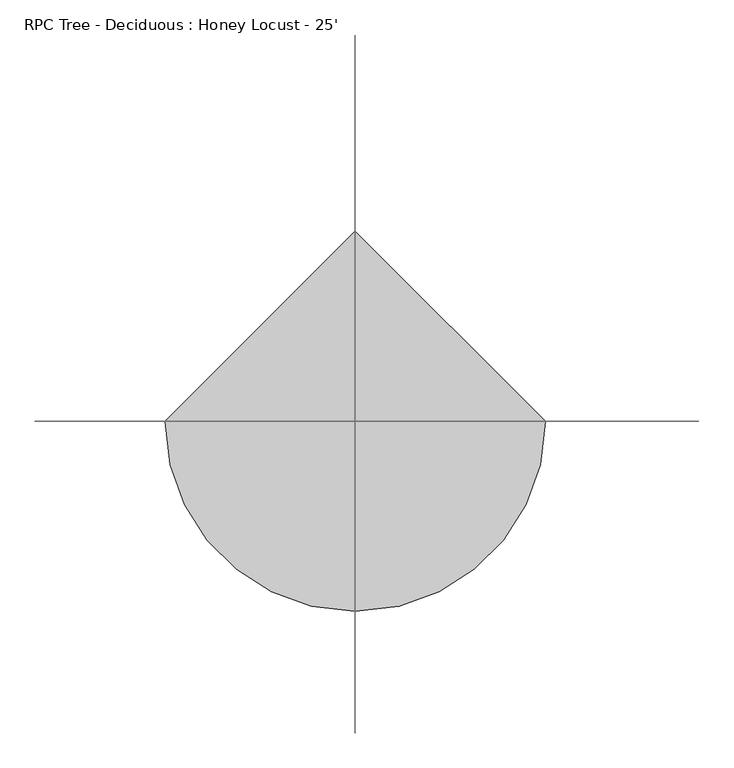
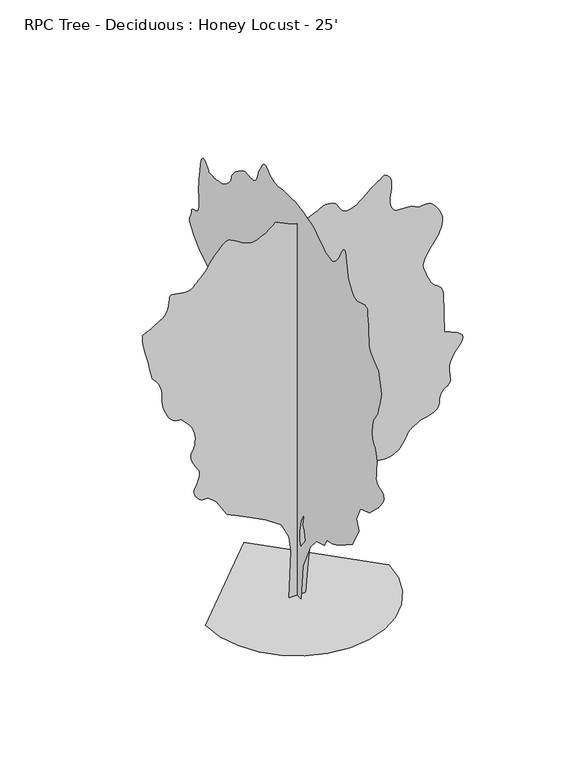
"""IFC4 building model written with IfcOpenShell, lengths in millimetres: geographic element geometry, RPC Tree - Deciduous : Honey Locust - 25'."""

from ifc_helpers import new_model, si_unit, origin, place, context, project, spatial, triangles, source, transform, mapped, element, save


def rpc_tree_deciduous_honey_locust_25_cc46a1f1(model_context):
    return source(origin(), model_context, "Body", "Tessellation", [
        triangles([(0.0017564, 138.2462219, 0.0), (0.0017564, -127.0105432, 0.0), (0.0017564, -184.6753374, 668.9082985), (0.0017564, -426.8668951, 1176.3566122), (0.0017564, -611.3926231, 1395.4822632), (0.0017564, -865.1155083, 1476.2135273), (0.0017564, -934.3152088, 1614.6078415), (0.0017564, -1118.8409369, 1660.7391827), (0.0017564, -1168.1321142, 1679.0297813), (0.0017564, -1234.9772346, 1712.4509972), (0.0017564, -1316.4476978, 1758.4833618), (0.0017564, -1409.6173016, 1814.6021748), (0.0017564, -1511.5651485, 1878.2849155), (0.0017564, -1619.3626385, 1947.0122612), (0.0017564, -1730.0862579, 2018.2590752), (0.0017564, -1937.6776566, 2398.8447109), (0.0017564, -1856.9463924, 2583.3806854), (0.0017564, -1983.8091431, 2848.632518), (0.0017564, -2272.1318058, 2952.4168808), (0.0017564, -2537.389016, 3206.1371498), (0.0017564, -2543.9089668, 3214.0110878), (0.0017564, -2561.3334846, 3235.1946785), (0.0017564, -2586.4031754, 3266.0558762), (0.0017564, -2615.9435234, 3302.9873428), (0.0017564, -2646.6774033, 3342.3317436), (0.0017564, -2675.3794304, 3380.4573235), (0.0017564, -2698.8489281, 3413.7311646), (0.0017564, -2714.4444878, 3444.5414932), (0.0017564, -2721.9882133, 3476.5453537), (0.0017564, -2721.8358971, 3508.1684235), (0.0017564, -2714.4444878, 3537.73377), (0.0017564, -2700.1950668, 3563.6926506), (0.0017564, -2679.4940048, 3584.4190018), (0.0017564, -2652.7226738, 3598.2620522), (0.0017564, -2621.3536583, 3608.345739), (0.0017564, -2588.1556847, 3619.6488281), (0.0017564, -2555.5675575, 3633.3648514), (0.0017564, -2526.024884, 3650.7129204), (0.0017564, -2501.9153091, 3672.9124374), (0.0017564, -2485.67444, 3701.157225), (0.0017564, -2479.7233498, 3736.6663948), (0.0017564, -2481.5749809, 3780.2273987), (0.0017564, -2486.0453476, 3831.0780739), (0.0017564, -2491.5266991, 3887.9740196), (0.0017564, -2496.4008202, 3949.6961243), (0.0017564, -2499.0579254, 4015.0755638), (0.0017564, -2497.8818344, 4082.8426483), (0.0017564, -2491.2575294, 4151.8544243), (0.0017564, -2477.5720276, 4213.7541344), (0.0017564, -2458.0368828, 4262.9284584), (0.0017564, -2435.2733013, 4302.24757), (0.0017564, -2411.9053963, 4334.4801956), (0.0017564, -2390.5542286, 4362.4965088), (0.0017564, -2373.8434753, 4389.0902344), (0.0017564, -2364.3947788, 4417.1062569), (0.0017564, -2359.5864967, 4450.1263344), (0.0017564, -2355.5860142, 4489.1913918), (0.0017564, -2353.1983692, 4533.3113731), (0.0017564, -2353.2315067, 4581.4694801), (0.0017564, -2356.4927902, 4632.6250786), (0.0017564, -2363.7901646, 4685.8128204), (0.0017564, -2375.9288132, 4740.016198), (0.0017564, -2392.0679443, 4787.9461212), (0.0017564, -2410.4271435, 4825.3601166), (0.0017564, -2430.3991802, 4855.916391), (0.0017564, -2451.3794403, 4883.2722794), (0.0017564, -2472.7636002, 4911.0089584), (0.0017564, -2493.9471909, 4942.7843445), (0.0017564, -2514.3232727, 4982.2051941), (0.0017564, -2534.0944496, 5031.4045166), (0.0017564, -2553.8659172, 5089.0626251), (0.0017564, -2573.6269203, 5153.8075104), (0.0017564, -2593.4135033, 5224.1654251), (0.0017564, -2613.1747971, 5298.7905212), (0.0017564, -2632.9360909, 5376.2096329), (0.0017564, -2652.7226738, 5455.0763306), (0.0017564, -2548.9127312, 5835.6443802), (0.0017564, -2410.52612, 5939.4537415), (0.0017564, -2376.165136, 5966.8602081), (0.0017564, -2343.2136589, 5995.5625259), (0.0017564, -2313.0867188, 6026.9059616), (0.0017564, -2287.1965839, 6062.1863663), (0.0017564, -2266.9553776, 6102.6995911), (0.0017564, -2253.772752, 6149.7659042), (0.0017564, -2249.0662079, 6204.705574), (0.0017564, -2247.7225399, 6269.3992996), (0.0017564, -2243.9556187, 6343.7709229), (0.0017564, -2238.1721054, 6426.2187973), (0.0017564, -2230.7756092, 6515.1186035), (0.0017564, -2222.1675591, 6608.8704391), (0.0017564, -2212.7518547, 6705.8220795), (0.0017564, -2202.9347214, 6804.4247818), (0.0017564, -2185.5179066, 6814.1270966), (0.0017564, -2167.3950302, 6822.8393555), (0.0017564, -2147.8598854, 6829.5453415), (0.0017564, -2126.2064106, 6833.2026764), (0.0017564, -2101.7285442, 6832.8218857), (0.0017564, -2073.7199341, 6827.4117508), (0.0017564, -2041.4746639, 6815.9560547), (0.0017564, -2006.8748863, 6801.3255524), (0.0017564, -1972.2775795, 6787.914743), (0.0017564, -1937.6776566, 6776.9165771), (0.0017564, -1903.077879, 6769.5501663), (0.0017564, -1868.4805721, 6767.0357849), (0.0017564, -1833.8806492, 6770.5663834), (0.0017564, -1799.2833424, 6781.3616547), (0.0017564, -1765.6919334, 6801.5546082), (0.0017564, -1733.9191635, 6831.4504578), (0.0017564, -1703.6576385, 6869.42314), (0.0017564, -1674.6050514, 6913.8221741), (0.0017564, -1646.4618565, 6963.0982361), (0.0017564, -1618.9257465, 7015.5746841), (0.0017564, -1591.689473, 7069.6766144), (0.0017564, -1522.4922432, 7484.8646439), (0.0017564, -1510.0182953, 7494.262326), (0.0017564, -1496.8382858, 7500.8665741), (0.0017564, -1482.2460079, 7501.8060516), (0.0017564, -1465.5354, 7494.262326), (0.0017564, -1446.0002552, 7475.4413818), (0.0017564, -1422.9345119, 7442.4974625), (0.0017564, -1395.6321087, 7392.5865555), (0.0017564, -1366.480545, 7335.9952423), (0.0017564, -1337.5296959, 7284.4588531), (0.0017564, -1307.5703327, 7237.3669601), (0.0017564, -1275.393663, 7194.085881), (0.0017564, -1239.7855167, 7154.0296051), (0.0017564, -1199.5366653, 7116.6156097), (0.0017564, -1153.4407871, 7081.2078873), (0.0017564, -1100.9873028, 7057.7133911), (0.0017564, -1043.0880753, 7054.1827927), (0.0017564, -980.6472645, 7067.2889694), (0.0017564, -914.5768787, 7093.7047989), (0.0017564, -845.7836214, 7130.1287384), (0.0017564, -775.1741959, 7173.2069229), (0.0017564, -703.6555235, 7219.6128113), (0.0017564, -659.2741482, 7251.5405136), (0.0017564, -615.4946983, 7282.3758408), (0.0017564, -572.9269114, 7311.0014191), (0.0017564, -532.1751838, 7336.2748764), (0.0017564, -493.8440932, 7357.1282547), (0.0017564, -458.5406522, 7372.4186005), (0.0017564, -426.8668951, 7381.0547012), (0.0017564, -379.7931333, 7391.6464966), (0.0017564, -304.4771091, 7410.7220764), (0.0017564, -210.8004869, 7434.013678), (0.0017564, -108.6519436, 7457.3308594), (0.0017564, -7.915369, 7476.3808594), (0.0017564, 81.5235032, 7486.9726547), (0.0017564, 149.779584, 7484.8646439), (0.0017564, 204.0816928, 7478.1336594), (0.0017564, 257.9799291, 7476.2541229), (0.0017564, 311.0709472, 7476.9907059), (0.0017564, 362.9529548, 7478.1336594), (0.0017564, 413.2194723, 7477.4732346), (0.0017564, 461.4692888, 7472.7485229), (0.0017564, 507.2984682, 7461.8015167), (0.0017564, 555.4821914, 7451.6666702), (0.0017564, 608.9110522, 7450.0156082), (0.0017564, 664.3541433, 7455.4513229), (0.0017564, 718.5906584, 7466.5000671), (0.0017564, 768.3873281, 7481.7909943), (0.0017564, 810.5182594, 7499.9265152), (0.0017564, 841.7526175, 7519.4590439), (0.0017564, 869.6950979, 7543.2081757), (0.0017564, 902.8827524, 7570.9704346), (0.0017564, 939.4967966, 7596.9293152), (0.0017564, 977.728838, 7615.2171524), (0.0017564, 1015.7551506, 7619.9924423), (0.0017564, 1051.7671967, 7605.3875198), (0.0017564, 1083.943939, 7565.5858795), (0.0017564, 1111.584185, 7516.9952408), (0.0017564, 1135.5896965, 7477.701709), (0.0017564, 1156.5725727, 7444.2496811), (0.0017564, 1175.132341, 7413.2114594), (0.0017564, 1191.8760138, 7381.1564392), (0.0017564, 1207.410676, 7344.6819214), (0.0017564, 1222.3407967, 7300.3334656), (0.0017564, 1236.6967518, 7254.9693741), (0.0017564, 1251.0554684, 7217.07285), (0.0017564, 1266.8236919, 7185.6526749), (0.0017564, 1285.4164524, 7159.6432159), (0.0017564, 1308.248489, 7138.103833), (0.0017564, 1336.7269833, 7119.9683121), (0.0017564, 1372.2666744, 7104.2710144), (0.0017564, 1413.6914715, 7095.1529663), (0.0017564, 1457.9408054, 7094.9239105), (0.0017564, 1503.6022625, 7099.7247803), (0.0017564, 1549.2612488, 7105.7447617), (0.0017564, 1593.5105827, 7109.1480423), (0.0017564, 1634.9353798, 7106.0999725), (0.0017564, 1672.1235168, 7092.7397415), (0.0017564, 1714.3205051, 7068.3051865), (0.0017564, 1768.2192501, 7035.5897415), (0.0017564, 1828.5747231, 6996.1944717), (0.0017564, 1890.1391338, 6951.7954376), (0.0017564, 1947.6700699, 6903.9419632), (0.0017564, 1995.9198864, 6854.2845291), (0.0017564, 2029.6434093, 6804.4247818), (0.0017564, 2047.5985634, 6762.5657089), (0.0017564, 2056.0720287, 6732.1873306), (0.0017564, 2061.1140175, 6707.879512), (0.0017564, 2068.7821541, 6684.1809586), (0.0017564, 2085.1219997, 6655.6315384), (0.0017564, 2116.1913242, 6616.7949554), (0.0017564, 2168.0377235, 6562.2360764), (0.0017564, 2230.1762272, 6507.9306702), (0.0017564, 2288.0754547, 6470.9736237), (0.0017564, 2341.7380222, 6447.5297058), (0.0017564, 2391.1637844, 6433.7881027), (0.0017564, 2436.3553574, 6425.8885849), (0.0017564, 2477.3077995, 6419.9959213), (0.0017564, 2514.0259071, 6412.2998795), (0.0017564, 2553.510125, 6405.0352066), (0.0017564, 2599.6366699, 6402.2161926), (0.0017564, 2647.7694878, 6402.6225632), (0.0017564, 2693.3117661, 6405.0352066), (0.0017564, 2731.5640823, 6408.2611725), (0.0017564, 2757.9293335, 6411.0807678), (0.0017564, 2767.7589661, 6412.2998795), (0.0017564, 2779.3922676, 6430.4609802), (0.0017564, 2809.9738312, 6472.8281616), (0.0017564, 2853.0775955, 6521.2403229), (0.0017564, 2902.2519196, 6557.5625244), (0.0017564, 2950.9945839, 6563.6075043), (0.0017564, 2992.9045258, 6521.2403229), (0.0017564, 3021.4792351, 6412.2998795), (0.0017564, 3039.1830963, 6281.2613663), (0.0017564, 3053.0770157, 6180.2965988), (0.0017564, 3063.5417839, 6102.7251709), (0.0017564, 3070.9584824, 6041.8916748), (0.0017564, 3075.7846413, 5991.1680267), (0.0017564, 3078.3751808, 5943.8482407), (0.0017564, 3079.1373436, 5893.3274872), (0.0017564, 3077.918232, 5838.9459229), (0.0017564, 3075.0986366, 5784.5899384), (0.0017564, 3071.8729614, 5730.2089554), (0.0017564, 3069.4600273, 5675.8273911), (0.0017564, 3069.0536568, 5621.4714066), (0.0017564, 3071.8729614, 5567.0904236), (0.0017564, 3079.1373436, 5512.7344391), (0.0017564, 3099.1779808, 5469.782991), (0.0017564, 3134.966494, 5444.6112717), (0.0017564, 3179.5942932, 5429.5238205), (0.0017564, 3226.2792343, 5416.8495941), (0.0017564, 3268.113018, 5398.9169678), (0.0017564, 3298.2376328, 5368.0816406), (0.0017564, 3309.7944855, 5316.6719879), (0.0017564, 3318.6843498, 5264.1193817), (0.0017564, 3338.4456436, 5228.1023941), (0.0017564, 3358.8164932, 5198.3588608), (0.0017564, 3369.5097359, 5164.551622), (0.0017564, 3360.2387901, 5116.4440933), (0.0017564, 3320.6912041, 5043.7235321), (0.0017564, 3240.6051041, 4936.0789398), (0.0017564, 3137.9128258, 4824.090136), (0.0017564, 3039.0560692, 4740.5243065), (0.0017564, 2946.4477684, 4678.5737274), (0.0017564, 2862.5264374, 4631.3298088), (0.0017564, 2789.7047195, 4591.9598282), (0.0017564, 2730.395549, 4553.5804848), (0.0017564, 2687.0124413, 4509.3590561), (0.0017564, 2658.1580978, 4464.7821259), (0.0017564, 2638.3970947, 4426.6568367), (0.0017564, 2624.0715157, 4390.1317406), (0.0017564, 2611.574604, 4350.4059677), (0.0017564, 2597.249025, 4302.5777824), (0.0017564, 2577.462442, 4241.8466057), (0.0017564, 2548.6333878, 4163.3859879), (0.0017564, 2517.7242279, 4078.1182274), (0.0017564, 2493.4823936, 3999.5052933), (0.0017564, 2474.7855698, 3926.4298119), (0.0017564, 2460.5312073, 3857.7988266), (0.0017564, 2449.6039673, 3792.521125), (0.0017564, 2440.8943245, 3729.4275925), (0.0017564, 2433.294643, 3667.4770134), (0.0017564, 2455.3521629, 3642.6102173), (0.0017564, 2476.2994308, 3616.9562599), (0.0017564, 2495.0267761, 3589.7021095), (0.0017564, 2510.4267082, 3560.0097359), (0.0017564, 2521.3894112, 3527.0913963), (0.0017564, 2526.8021622, 3490.1343498), (0.0017564, 2525.5600868, 3448.3514351), (0.0017564, 2526.3652702, 3406.9748909), (0.0017564, 2533.4264671, 3370.2718987), (0.0017564, 2538.8723557, 3335.7786552), (0.0017564, 2534.8385902, 3301.0569374), (0.0017564, 2513.4544304, 3263.7443893), (0.0017564, 2466.850589, 3221.3772079), (0.0017564, 2387.1633018, 3171.5424591), (0.0017564, 2299.4063038, 3131.0039452), (0.0017564, 2230.2092194, 3111.2173622), (0.0017564, 2174.1235439, 3101.9464165), (0.0017564, 2125.7061504, 3092.878656), (0.0017564, 2079.5060635, 3073.7016289), (0.0017564, 2030.0803013, 3034.1540428), (0.0017564, 1971.9778885, 2963.9484444), (0.0017564, 1918.922406, 2886.046804), (0.0017564, 1885.02869, 2826.5091591), (0.0017564, 1865.4579369, 2779.671611), (0.0017564, 1855.3716339, 2739.8952599), (0.0017564, 1849.9258907, 2701.5159164), (0.0017564, 1844.2769623, 2658.9202606), (0.0017564, 1833.5835743, 2606.4438126), (0.0017564, 1823.3625412, 2556.2026932), (0.0017564, 1818.1834969, 2520.8993248), (0.0017564, 1811.7953693, 2495.6822594), (0.0017564, 1797.9422905, 2475.7102226), (0.0017564, 1770.3705723, 2456.1393242), (0.0017564, 1722.8269627, 2432.1339581), (0.0017564, 1649.0577736, 2398.8447109), (0.0017564, 1567.2851486, 2366.9372108), (0.0017564, 1497.6180347, 2346.9297112), (0.0017564, 1436.6226299, 2333.7851646), (0.0017564, 1380.8747246, 2322.4516994), (0.0017564, 1326.9429874, 2307.8950298), (0.0017564, 1271.3957966, 2285.0629932), (0.0017564, 1210.806617, 2248.9188332), (0.0017564, 1144.870816, 2202.0812851), (0.0017564, 1075.9099091, 2151.0044609), (0.0017564, 1004.4242289, 2096.4021252), (0.0017564, 930.9242821, 2038.9727818), (0.0017564, 855.9105469, 1979.4251083), (0.0017564, 779.8858995, 1918.4651665), (0.0017564, 703.3583033, 1856.7991631), (0.0017564, 276.64129, 1533.8765774), (0.0017564, 149.779584, 1314.7509991), (0.0017564, 115.1805058, 1141.7593054), (0.0017564, 103.6476433, 876.5023132), (0.0020752, -103.9448272, 980.2967772), (0.0020752, -80.8791112, 1107.1595278), (0.0020752, -80.8791112, 1268.6195126), (0.0020752, -127.0105432, 1499.2792706), (0.0020752, -230.8067694, 1706.8706692), (0.0020752, -184.6753374, 1453.147784), (0.0020752, -230.8067694, 1372.4165199), (0.0020752, -265.4043305, 1199.4223555), (154.7882082, 0.0004434, 0.0162828), (-145.0671264, 0.0004434, 0.0162828), (-110.4685569, 0.0003925, 876.5175739), (-145.0671264, 0.000378, 1164.8403093), (-283.4611681, 0.0003635, 1441.6288651), (-560.2523217, 0.0003489, 1637.6887001), (-963.9036644, 0.0003344, 1845.2827148), (-1263.7605068, 0.0003271, 1983.677029), (-1459.8203419, 0.0003126, 2295.065435), (-1609.7462196, 0.000298, 2421.9281857), (-1636.8810459, 0.0003053, 2419.6396626), (-1663.7135651, 0.0003053, 2418.4637169), (-1689.9389992, 0.0003053, 2419.5050777), (-1715.2578026, 0.000298, 2423.8764679), (-1739.3649067, 0.000298, 2432.6877033), (-1761.9606205, 0.000298, 2447.0436584), (-1782.7404568, 0.000298, 2468.0595268), (-1802.9155334, 0.000298, 2493.4774521), (-1822.6843849, 0.000298, 2520.3098259), (-1840.2357845, 0.0002908, 2548.5572296), (-1853.7537094, 0.0002908, 2578.199025), (-1861.4193752, 0.0002908, 2609.2886971), (-1861.4193752, 0.0002908, 2641.7497971), (-1851.9375412, 0.0002835, 2675.6587738), (-1833.5784874, 0.0002835, 2714.1904335), (-1810.985099, 0.0002835, 2759.3769196), (-1788.3893852, 0.0002762, 2809.4148537), (-1770.0301861, 0.0002762, 2862.4755684), (-1760.1445976, 0.000269, 2916.7298149), (-1762.9689892, 0.000269, 2970.4000854), (-1782.7404568, 0.000269, 3021.631842), (-1812.8012672, 0.0002617, 3069.7646599), (-1842.4557072, 0.0002617, 3115.6624397), (-1869.8928406, 0.0002544, 3159.9347374), (-1893.2963539, 0.0002544, 3203.2161072), (-1910.8477535, 0.0002544, 3246.0658173), (-1920.7308712, 0.0002471, 3289.1442924), (-1921.134771, 0.0002471, 3333.0355087), (-1913.6366821, 0.0002471, 3370.6526894), (-1902.1049732, 0.0002399, 3398.1864738), (-1888.1503017, 0.0002399, 3421.0972847), (-1873.3903015, 0.0002399, 3444.7952568), (-1859.43563, 0.0002399, 3474.7419754), (-1847.9014503, 0.0002399, 3516.397863), (-1840.4059776, 0.0002326, 3575.2242142), (-1839.1614315, 0.0002253, 3640.3751793), (-1844.5740372, 0.0002253, 3698.2870514), (-1855.534124, 0.0002253, 3750.1283638), (-1870.9342014, 0.0002181, 3797.143808), (-1889.6641628, 0.0002181, 3840.5016266), (-1910.6114307, 0.0002181, 3881.4718002), (-1932.6688053, 0.0002108, 3921.1972824), (-2094.1288628, 0.0002035, 4094.1966064), (-2131.1822697, 0.0002035, 4094.6791351), (-2168.1342293, 0.0002035, 4097.9556793), (-2204.8854744, 0.0002035, 4106.8964127), (-2241.3344124, 0.0002035, 4124.3209305), (-2277.3769798, 0.0001963, 4153.0482468), (-2312.9191418, 0.0001963, 4195.8726677), (-2347.8542187, 0.000189, 4255.6640762), (-2378.9895275, 0.000189, 4321.6024933), (-2403.4675392, 0.0001817, 4382.0799065), (-2421.6893921, 0.0001817, 4438.7470871), (-2434.0643635, 0.0001817, 4493.1792297), (-2440.9908302, 0.0001745, 4547.0018166), (-2442.8729828, 0.0001745, 4601.8403297), (-2440.1170464, 0.0001672, 4659.3205421), (-2439.9138611, 0.0001672, 4717.8166809), (-2448.3874718, 0.0001599, 4774.3062561), (-2464.3234177, 0.0001599, 4828.1797119), (-2486.5177025, 0.0001527, 4878.801622), (-2513.751796, 0.0001527, 4925.6138809), (-2544.8234459, 0.0001527, 4967.9810623), (-2578.5039482, 0.0001454, 5005.2933197), (-2606.1136002, 0.0001454, 5036.2053864), (-2622.8268242, 0.0001454, 5064.6786484), (-2633.2915924, 0.0001454, 5098.2068344), (-2642.1308784, 0.0001381, 5144.2313507), (-2653.9926544, 0.0001381, 5210.2459259), (-2673.5251831, 0.0001308, 5303.6669678), (-2705.3767273, 0.0001236, 5432.0132034), (-2739.5397583, 0.0001163, 5564.8295151), (-2764.0251823, 0.000109, 5669.807991), (-2780.4334831, 0.0001018, 5751.5704422), (-2790.3651443, 0.0001018, 5814.7910019), (-2795.4959358, 9.45e-05, 5864.0920624), (-2797.3754723, 9.45e-05, 5904.0971786), (-2797.6295265, 9.45e-05, 5939.4537415), (-2780.0526924, 9.45e-05, 5947.0736252), (-2760.7486382, 9.45e-05, 5955.7608856), (-2738.0157234, 8.72e-05, 5966.7078918), (-2710.1520172, 8.72e-05, 5980.9576035), (-2675.4047195, 8.72e-05, 5999.6518112), (-2632.0977699, 8.72e-05, 6023.8834717), (-2578.5039482, 8.72e-05, 6054.794957), (-2522.6948547, 8e-05, 6086.4941849), (-2473.739122, 8e-05, 6114.9674469), (-2431.4405411, 8e-05, 6144.0761353), (-2395.5985428, 8e-05, 6177.5787415), (-2366.0102325, 7.27e-05, 6219.387236), (-2342.4746052, 7.27e-05, 6273.2856903), (-2324.7886208, 6.54e-05, 6343.110498), (-2314.1282249, 6.54e-05, 6412.6556717), (-2308.7154739, 5.82e-05, 6464.4205353), (-2303.9071918, 5.82e-05, 6500.4631027), (-2295.0629642, 5.82e-05, 6522.7896469), (-2277.5471729, 5.82e-05, 6533.4320206), (-2246.7141712, 5.82e-05, 6534.3720795), (-2197.9258701, 5.82e-05, 6527.641095), (-2140.092627, 5.82e-05, 6517.4300903), (-2085.4878204, 5.82e-05, 6508.0068283), (-2034.5150597, 5.82e-05, 6501.6060562), (-1987.575919, 5.82e-05, 6500.4631027), (-1945.0767689, 5.82e-05, 6506.7877167), (-1907.4187477, 5.82e-05, 6522.7896469), (-1875.0032845, 5.82e-05, 6550.7042221), (-1844.541045, 5.09e-05, 6583.0894547), (-1812.0595974, 5.09e-05, 6613.4422531), (-1776.9567982, 5.09e-05, 6645.4205338), (-1738.6257076, 5.09e-05, 6682.6572144), (-1696.4617115, 4.36e-05, 6728.7578888), (-1649.8604862, 4.36e-05, 6787.3560562), (-1598.2146561, 3.63e-05, 6862.1078888), (-1546.1980637, 2.91e-05, 6938.7142593), (-1498.4181313, 2.91e-05, 7002.036557), (-1454.1714134, 2.91e-05, 7054.2589508), (-1412.7466164, 2.18e-05, 7097.5911896), (-1373.4401493, 2.18e-05, 7134.268602), (-1335.5459507, 2.18e-05, 7166.5265167), (-1298.3578136, 1.45e-05, 7196.5496841), (-1288.0707962, 1.45e-05, 7208.5129074), (-1275.3606709, 1.45e-05, 7218.1646439), (-1257.8092712, 1.45e-05, 7223.193988), (-1232.9934895, 1.45e-05, 7221.2382935), (-1198.4952318, 1.45e-05, 7210.0116531), (-1151.8939339, 1.45e-05, 7187.1770004), (-1090.7663424, 2.18e-05, 7150.4228485), (-1026.7456861, 2.18e-05, 7109.5544128), (-971.2010387, 2.18e-05, 7076.382019), (-921.3027763, 2.91e-05, 7051.4649353), (-874.2290508, 2.91e-05, 7035.4374252), (-827.1577961, 2.91e-05, 7028.858757), (-777.2595337, 2.91e-05, 7032.3893555), (-721.7123428, 2.91e-05, 7046.6134872), (-664.755427, 2.18e-05, 7068.7365555), (-612.0327003, 2.18e-05, 7095.1018066), (-562.8405722, 2.18e-05, 7124.9976563), (-516.4729082, 2.18e-05, 7157.7131012), (-472.226154, 1.45e-05, 7192.5615555), (-429.3891249, 1.45e-05, 7228.8075989), (-387.2581573, 1.45e-05, 7265.7390656), (-168.1328515, 2.18e-05, 7161.9547028), (-133.3996518, 2.18e-05, 7144.8603973), (-97.8597517, 2.18e-05, 7129.1125214), (-60.7056832, 2.18e-05, 7115.9551849), (-21.1306711, 2.18e-05, 7106.7348175), (21.6722237, 2.18e-05, 7102.77285), (68.5100806, 2.18e-05, 7105.3633896), (120.1896296, 2.18e-05, 7115.8284485), (179.9390167, 2.18e-05, 7135.6656097), (246.5473965, 2.18e-05, 7162.9709198), (314.1646537, 1.45e-05, 7193.9079849), (376.9406911, 1.45e-05, 7224.6165756), (429.0233405, 1.45e-05, 7251.3120392), (464.5629953, 1.45e-05, 7270.1585632), (477.7100126, 1.45e-05, 7277.2703384), (487.5271096, 1.45e-05, 7279.4550888), (513.8897447, 1.45e-05, 7283.4682159), (552.1522711, 1.45e-05, 7285.4494904), (597.6791797, 1.45e-05, 7281.5886795), (645.8273672, 1.45e-05, 7268.0249725), (691.9587811, 1.45e-05, 7240.9737167), (731.4328978, 1.45e-05, 7196.5496841), (761.0238968, 2.18e-05, 7148.2642593), (783.1472557, 2.18e-05, 7111.0787384), (801.640967, 2.18e-05, 7083.3670578), (820.3353928, 2.18e-05, 7063.5298965), (843.065764, 2.91e-05, 7049.9406097), (873.6625883, 2.91e-05, 7040.9998764), (915.9611692, 2.91e-05, 7035.081633), (967.9092339, 2.91e-05, 7039.3999741), (1023.6901314, 2.18e-05, 7059.6435059), (1081.4903097, 2.18e-05, 7091.9775787), (1139.4911299, 2.18e-05, 7132.5925415), (1195.8764963, 1.45e-05, 7177.6520004), (1248.8354004, 1.45e-05, 7223.3207245), (1296.5467323, 1.45e-05, 7265.7390656), (1340.3591743, 7.3e-06, 7303.2803787), (1382.9600624, 7.3e-06, 7337.1637756), (1424.5524364, 7.3e-06, 7368.0246826), (1465.3373016, 7.3e-06, 7396.4723648), (1505.5174072, 0.0, 7423.1172501), (1545.2937584, 0.0, 7448.5168625), (1584.8695404, 0.0, 7473.3327896), (1611.8696365, 0.0, 7460.5568253), (1637.7599167, 0.0, 7445.2658981), (1661.4301289, 0.0, 7424.9206284), (1681.7729279, 7.3e-06, 7397.0060532), (1697.6758816, 7.3e-06, 7359.0327896), (1708.0339703, 7.3e-06, 7308.4108795), (1711.732291, 1.45e-05, 7242.6759384), (1708.6384392, 2.18e-05, 7173.2069229), (1701.1073582, 2.18e-05, 7112.0182159), (1691.7602543, 2.18e-05, 7057.4843353), (1683.2181885, 2.91e-05, 7007.9797989), (1678.1077446, 2.91e-05, 6961.9297028), (1679.0501289, 3.63e-05, 6917.6829849), (1688.6665478, 3.63e-05, 6873.639743), (1703.4950031, 3.63e-05, 6833.8631012), (1718.3209877, 4.36e-05, 6802.5452454), (1733.1494431, 4.36e-05, 6778.3135849), (1747.9780437, 4.36e-05, 6759.7205338), (1762.8064991, 4.36e-05, 6745.3440857), (1777.6324837, 4.36e-05, 6733.8128128), (1792.460939, 4.36e-05, 6723.7035461), (2069.2520382, 4.36e-05, 6712.1716919), (2207.6463524, 5.09e-05, 6642.9823105), (2217.499094, 5.09e-05, 6645.8524841), (2244.0954357, 5.09e-05, 6651.9742035), (2282.9953869, 5.09e-05, 6657.485495), (2329.7669506, 5.09e-05, 6658.5778702), (2379.9675201, 5.09e-05, 6651.3899368), (2429.1595757, 5.09e-05, 6632.0858826), (2472.9034172, 5.09e-05, 6596.8304764), (2512.6797684, 5.82e-05, 6549.0025818), (2551.0463219, 5.82e-05, 6495.1035461), (2585.1840637, 6.54e-05, 6436.1501678), (2612.2350288, 6.54e-05, 6373.1836624), (2629.4307816, 7.27e-05, 6307.1690872), (2633.9011482, 7.27e-05, 6239.1482391), (2622.8268242, 8e-05, 6170.111174), (2602.049604, 8e-05, 6105.620343), (2579.4690056, 8.72e-05, 6049.6132965), (2555.3390831, 8.72e-05, 6000.6680283), (2530.0304535, 8.72e-05, 5957.360788), (2503.8024033, 9.45e-05, 5918.2701508), (2476.9726456, 9.45e-05, 5882.0246887), (2449.837674, 9.45e-05, 5847.2012329), (2408.2121624, 0.0001018, 5785.5299973), (2368.9058407, 0.0001018, 5724.5703461), (2334.2399334, 0.000109, 5665.0327011), (2306.5336304, 0.000109, 5607.603067), (2288.1084469, 0.0001163, 5552.9930283), (2281.2834274, 0.0001163, 5501.9141693), (2288.3777618, 0.0001236, 5455.0763306), (2303.2722015, 0.0001236, 5411.8202499), (2318.5706863, 0.0001236, 5370.1390732), (2334.6768253, 0.0001308, 5328.8892654), (2351.9919022, 0.0001308, 5286.8267166), (2370.922578, 0.0001308, 5242.7578949), (2391.869846, 0.0001381, 5195.4375275), (2415.2378963, 0.0001381, 5143.6982437), (2445.5678764, 0.0001454, 5097.4190918), (2484.1684273, 0.0001454, 5063.0531662), (2526.5989769, 0.0001454, 5034.1479538), (2568.4199707, 0.0001454, 5004.2265244), (2605.2247009, 0.0001527, 4966.8381088), (2632.5041405, 0.0001527, 4915.5301941), (2645.8899513, 0.0001599, 4843.8258499), (2668.9530785, 0.0002035, 4105.72817), (2899.6102203, 0.0002108, 4001.9438072), (2935.957711, 0.0002108, 3979.3123398), (2967.9871513, 0.0002108, 3954.3696762), (2991.3043327, 0.0002108, 3924.7787498), (3001.6420738, 0.0002108, 3888.2280739), (2994.6061661, 0.0002181, 3842.381163), (2965.9041389, 0.0002181, 3784.9518196), (2911.1417839, 0.0002253, 3713.6032677), (2850.7916885, 0.0002326, 3637.2509514), (2806.7987343, 0.0002326, 3565.9279793), (2777.1063606, 0.0002399, 3499.049794), (2759.707132, 0.0002399, 3436.0068398), (2752.6206459, 0.0002471, 3376.1901421), (2753.7891792, 0.0002471, 3319.0145622), (2761.2311668, 0.0002544, 3263.8205475), (2769.4861862, 0.0002544, 3214.1381149), (2773.7280785, 0.0002544, 3172.7107018), (2772.7374413, 0.0002617, 3137.9384056), (2765.2698738, 0.0002617, 3108.2201614), (2750.1315536, 0.0002617, 3081.9313591), (2726.1283676, 0.0002617, 3057.4456444), (2692.0162056, 0.0002617, 3033.1634056), (2656.5834846, 0.000269, 3007.7126335), (2628.8212257, 0.000269, 2980.6616684), (2607.8916893, 0.000269, 2951.756456), (2593.0327126, 0.000269, 2920.8699692), (2583.4315544, 0.0002762, 2887.7484444), (2578.249894, 0.0002762, 2852.2139854), (2576.7002792, 0.0002762, 2814.0378273), (2574.4905304, 0.0002835, 2776.5473831), (2567.4293335, 0.0002835, 2742.8924606), (2554.9071327, 0.0002835, 2712.6663986), (2536.3501259, 0.0002835, 2685.4631172), (2511.1330605, 0.0002908, 2660.9012444), (2478.6539383, 0.0002908, 2638.5238312), (2438.3036396, 0.0002908, 2617.9753761), (2396.3758209, 0.0002908, 2601.9734459), (2358.4816223, 0.0002908, 2591.6357048), (2323.0080608, 0.0002908, 2584.0916885), (2288.3421535, 0.0002908, 2576.5735428), (2252.8710629, 0.0002908, 2566.2102219), (2214.9768642, 0.0002908, 2550.2082916), (2173.0465748, 0.000298, 2525.7225769), (2134.3801849, 0.000298, 2501.648465), (2105.1956291, 0.000298, 2485.6439186), (2082.2644707, 0.000298, 2473.0685234), (2062.3585636, 0.000298, 2459.2838997), (2042.2519421, 0.000298, 2439.6473076), (2018.7163147, 0.0003053, 2409.5203674), (1988.5207741, 0.0003053, 2364.2626648), (1957.3856106, 0.0003053, 2310.7346821), (1930.083062, 0.0003126, 2259.4242966), (1901.9730045, 0.0003126, 2211.1414879), (1868.4170586, 0.0003198, 2166.6889687), (1824.7748096, 0.0003198, 2126.8796253), (1766.4030819, 0.0003198, 2092.5158798), (1688.6665478, 0.0003198, 2064.4058224), (1611.2981598, 0.0003271, 2049.7144226), (1552.6928707, 0.0003271, 2049.9481293), (1506.1906219, 0.0003198, 2057.4462181), (1465.1365871, 0.0003198, 2064.5404072), (1422.8709984, 0.0003198, 2063.5676468), (1372.7390293, 0.0003271, 2046.8544228), (1308.0784412, 0.0003271, 2006.7427723), (1236.0922829, 0.0003271, 1957.583709), (1168.5411009, 0.0003344, 1917.1011509), (1105.630406, 0.0003344, 1882.6715664), (1047.5635288, 0.0003344, 1851.6708424), (994.5385677, 0.0003344, 1821.4753017), (946.7611788, 0.0003416, 1789.4663544), (904.4270622, 0.0003416, 1753.0174164), (863.5407497, 0.0003416, 1713.1393272), (820.2337275, 0.0003489, 1672.6569145), (774.9100405, 0.0003489, 1631.6714802), (727.9708998, 0.0003489, 1590.2796753), (679.8201324, 0.0003562, 1548.5857086), (630.8642544, 0.0003562, 1506.6908821), (581.50702, 0.0003562, 1464.6946083), (339.3157348, 0.000378, 1176.3718729), (235.5192361, 0.0003925, 899.5832445), (200.9196402, 0.0004143, 542.0633883), (-1658.5903313, 0.0, 0.0172132), (-1614.7424263, -380.0394845, 0.0172132), (-1489.866037, -729.0453255, 0.0172132), (-1293.9560474, -1037.0174429, 0.0172132), (-1037.0174429, -1293.9560474, 0.0172132), (-729.0453255, -1489.866037, 0.0172132), (-380.0394845, -1614.7424263, 0.0172132), (7.25e-05, -1658.5903313, 0.0172132), (380.0394845, -1614.7424263, 0.0172132), (729.0453255, -1489.866037, 0.0172132), (1037.0174429, -1293.9560474, 0.0172132), (1293.9560474, -1037.0174429, 0.0172132), (1489.866037, -729.0453255, 0.0172132), (1614.7424263, -380.0394845, 0.0172132), (1658.5903313, 0.0001454, 0.0172132), (-0.0002175, 1658.5903313, 0.0172132)], [[328, 1, 329], [327, 328, 329], [327, 329, 330], [329, 1, 2], [329, 2, 3], [329, 3, 4], [336, 329, 4], [327, 330, 331], [326, 327, 331], [326, 331, 332], [325, 326, 332], [335, 336, 4], [335, 4, 5], [325, 332, 333], [334, 335, 5], [333, 334, 5], [333, 5, 6], [333, 6, 7], [324, 325, 333], [91, 92, 93], [223, 224, 225], [222, 223, 225], [222, 225, 226], [221, 222, 226], [220, 221, 226], [220, 226, 227], [219, 220, 227], [219, 227, 228], [15, 16, 17], [91, 93, 94], [91, 94, 95], [91, 95, 96], [91, 96, 97], [91, 97, 98], [91, 98, 99], [91, 99, 100], [90, 91, 100], [90, 100, 101], [90, 101, 102], [89, 90, 102], [89, 102, 103], [88, 89, 103], [88, 103, 104], [218, 219, 228], [14, 15, 17], [218, 228, 229], [217, 218, 229], [216, 217, 229], [216, 229, 230], [215, 216, 230], [215, 230, 231], [214, 215, 231], [214, 231, 232], [214, 232, 233], [214, 233, 234], [213, 214, 234], [213, 234, 235], [113, 114, 115], [113, 115, 116], [113, 116, 117], [113, 117, 118], [113, 118, 119], [113, 119, 120], [113, 120, 121], [113, 121, 122], [113, 122, 123], [113, 123, 124], [113, 124, 125], [113, 125, 126], [113, 126, 127], [112, 113, 127], [112, 127, 128], [111, 112, 128], [110, 111, 128], [213, 235, 236], [87, 88, 104], [87, 104, 105], [212, 213, 236], [110, 128, 129], [109, 110, 129], [212, 236, 237], [211, 212, 237], [210, 211, 237], [86, 87, 105], [210, 237, 238], [209, 210, 238], [85, 86, 105], [76, 77, 78], [75, 76, 78], [13, 14, 17], [209, 238, 239], [85, 105, 106], [208, 209, 239], [74, 75, 78], [108, 109, 129], [74, 78, 79], [73, 74, 79], [84, 85, 106], [73, 79, 80], [72, 73, 80], [71, 72, 80], [208, 239, 240], [70, 71, 80], [69, 70, 80], [68, 69, 80], [67, 68, 80], [66, 67, 80], [65, 66, 80], [65, 80, 81], [64, 65, 81], [12, 13, 17], [245, 246, 247], [244, 245, 247], [243, 244, 247], [243, 247, 248], [64, 81, 82], [63, 64, 82], [242, 243, 248], [323, 324, 333], [167, 168, 169], [167, 169, 170], [166, 167, 170], [166, 170, 171], [165, 166, 171], [164, 165, 171], [164, 171, 172], [163, 164, 172], [163, 172, 173], [163, 173, 174], [162, 163, 174], [162, 174, 175], [162, 175, 176], [162, 176, 177], [161, 162, 177], [161, 177, 178], [161, 178, 179], [160, 161, 179], [160, 179, 180], [159, 160, 180], [159, 180, 181], [158, 159, 181], [11, 12, 17], [250, 251, 252], [249, 250, 252], [249, 252, 253], [248, 249, 253], [242, 248, 253], [242, 253, 254], [242, 254, 255], [241, 242, 255], [241, 255, 256], [241, 256, 257], [241, 257, 258], [241, 258, 259], [240, 241, 259], [208, 240, 259], [208, 259, 260], [208, 260, 261], [207, 208, 261], [206, 207, 261], [206, 261, 262], [206, 262, 263], [205, 206, 263], [205, 263, 264], [204, 205, 264], [204, 264, 265], [204, 265, 266], [204, 266, 267], [204, 267, 268], [204, 268, 269], [203, 204, 269], [10, 11, 17], [9, 10, 17], [8, 9, 17], [7, 8, 17], [333, 7, 17], [323, 333, 17], [322, 323, 17], [322, 17, 18], [321, 322, 18], [320, 321, 18], [319, 320, 18], [318, 319, 18], [317, 318, 18], [316, 317, 18], [315, 316, 18], [203, 269, 270], [314, 315, 18], [18, 19, 20], [314, 18, 20], [314, 20, 21], [314, 21, 22], [314, 22, 23], [314, 23, 24], [314, 24, 25], [314, 25, 26], [314, 26, 27], [314, 27, 28], [314, 28, 29], [314, 29, 30], [314, 30, 31], [314, 31, 32], [314, 32, 33], [314, 33, 34], [314, 34, 35], [314, 35, 36], [314, 36, 37], [314, 37, 38], [314, 38, 39], [314, 39, 40], [314, 40, 41], [314, 41, 42], [314, 42, 43], [314, 43, 44], [314, 44, 45], [314, 45, 46], [314, 46, 47], [314, 47, 48], [314, 48, 49], [314, 49, 50], [314, 50, 51], [314, 51, 52], [314, 52, 53], [314, 53, 54], [314, 54, 55], [314, 55, 56], [314, 56, 57], [314, 57, 58], [314, 58, 59], [314, 59, 60], [314, 60, 61], [314, 61, 62], [313, 314, 62], [312, 313, 62], [311, 312, 62], [310, 311, 62], [309, 310, 62], [308, 309, 62], [307, 308, 62], [306, 307, 62], [305, 306, 62], [304, 305, 62], [303, 304, 62], [302, 303, 62], [301, 302, 62], [300, 301, 62], [299, 300, 62], [298, 299, 62], [297, 298, 62], [296, 297, 62], [295, 296, 62], [294, 295, 62], [294, 62, 63], [294, 63, 82], [294, 82, 83], [294, 83, 84], [294, 84, 106], [294, 106, 107], [294, 107, 108], [294, 108, 129], [294, 129, 130], [294, 130, 131], [294, 131, 132], [294, 132, 133], [294, 133, 134], [294, 134, 135], [294, 135, 136], [294, 136, 137], [294, 137, 138], [294, 138, 139], [294, 139, 140], [294, 140, 141], [294, 141, 142], [294, 142, 143], [294, 143, 144], [294, 144, 145], [294, 145, 146], [294, 146, 147], [294, 147, 148], [294, 148, 149], [294, 149, 150], [294, 150, 151], [294, 151, 152], [294, 152, 153], [294, 153, 154], [294, 154, 155], [294, 155, 156], [294, 156, 157], [294, 157, 158], [294, 158, 181], [294, 181, 182], [294, 182, 183], [294, 183, 184], [294, 184, 185], [293, 294, 185], [293, 185, 186], [293, 186, 187], [292, 293, 187], [292, 187, 188], [292, 188, 189], [292, 189, 190], [292, 190, 191], [292, 191, 192], [292, 192, 193], [292, 193, 194], [292, 194, 195], [292, 195, 196], [292, 196, 197], [292, 197, 198], [292, 198, 199], [292, 199, 200], [292, 200, 201], [292, 201, 202], [292, 202, 203], [292, 203, 270], [292, 270, 271], [292, 271, 272], [292, 272, 273], [292, 273, 274], [292, 274, 275], [291, 292, 275], [290, 291, 275], [289, 290, 275], [289, 275, 276], [289, 276, 277], [289, 277, 278], [289, 278, 279], [289, 279, 280], [289, 280, 281], [289, 281, 282], [289, 282, 283], [288, 289, 283], [288, 283, 284], [287, 288, 284], [286, 287, 284], [285, 286, 284], [337, 338, 339], [677, 337, 339], [676, 677, 339], [676, 339, 340], [675, 676, 340], [423, 424, 425], [486, 487, 488], [675, 340, 341], [674, 675, 341], [529, 530, 531], [485, 486, 488], [484, 485, 488], [423, 425, 426], [529, 531, 532], [673, 674, 341], [673, 341, 342], [672, 673, 342], [671, 672, 342], [670, 671, 342], [669, 670, 342], [668, 669, 342], [667, 668, 342], [529, 532, 533], [528, 529, 533], [528, 533, 534], [528, 534, 535], [528, 535, 536], [527, 528, 536], [527, 536, 537], [526, 527, 537], [526, 537, 538], [525, 526, 538], [525, 538, 539], [524, 525, 539], [524, 539, 540], [523, 524, 540], [523, 540, 541], [522, 523, 541], [522, 541, 542], [521, 522, 542], [521, 542, 543], [520, 521, 543], [519, 520, 543], [519, 543, 544], [519, 544, 545], [518, 519, 545], [518, 545, 546], [517, 518, 546], [517, 546, 547], [422, 423, 426], [422, 426, 427], [441, 442, 443], [441, 443, 444], [440, 441, 444], [440, 444, 445], [439, 440, 445], [439, 445, 446], [438, 439, 446], [438, 446, 447], [438, 447, 448], [437, 438, 448], [437, 448, 449], [666, 667, 342], [421, 422, 427], [421, 427, 428], [421, 428, 429], [420, 421, 429], [420, 429, 430], [419, 420, 430], [419, 430, 431], [418, 419, 431], [418, 431, 432], [418, 432, 433], [417, 418, 433], [417, 433, 434], [416, 417, 434], [483, 484, 488], [436, 437, 449], [343, 344, 345], [666, 342, 343], [666, 343, 345], [665, 666, 345], [664, 665, 345], [663, 664, 345], [662, 663, 345], [661, 662, 345], [660, 661, 345], [659, 660, 345], [659, 345, 346], [517, 547, 548], [483, 488, 489], [416, 434, 435], [415, 416, 435], [482, 483, 489], [482, 489, 490], [436, 449, 450], [658, 659, 346], [414, 415, 435], [600, 601, 602], [599, 600, 602], [599, 602, 603], [598, 599, 603], [597, 598, 603], [597, 603, 604], [596, 597, 604], [596, 604, 605], [596, 605, 606], [596, 606, 607], [596, 607, 608], [516, 517, 548], [516, 548, 549], [413, 414, 435], [412, 413, 435], [411, 412, 435], [410, 411, 435], [409, 410, 435], [408, 409, 435], [407, 408, 435], [407, 435, 436], [407, 436, 450], [407, 450, 451], [406, 407, 451], [405, 406, 451], [405, 451, 452], [404, 405, 452], [404, 452, 453], [404, 453, 454], [404, 454, 455], [404, 455, 456], [551, 552, 553], [482, 490, 491], [481, 482, 491], [404, 456, 457], [467, 468, 469], [467, 469, 470], [466, 467, 470], [466, 470, 471], [466, 471, 472], [465, 466, 472], [465, 472, 473], [464, 465, 473], [463, 464, 473], [463, 473, 474], [462, 463, 474], [461, 462, 474], [461, 474, 475], [460, 461, 475], [459, 460, 475], [459, 475, 476], [458, 459, 476], [458, 476, 477], [457, 458, 477], [404, 457, 477], [404, 477, 478], [404, 478, 479], [404, 479, 480], [403, 404, 480], [403, 480, 481], [403, 481, 491], [403, 491, 492], [403, 492, 493], [402, 403, 493], [401, 402, 493], [400, 401, 493], [399, 400, 493], [398, 399, 493], [397, 398, 493], [396, 397, 493], [395, 396, 493], [394, 395, 493], [393, 394, 493], [392, 393, 493], [391, 392, 493], [390, 391, 493], [389, 390, 493], [388, 389, 493], [387, 388, 493], [386, 387, 493], [386, 493, 494], [385, 386, 494], [384, 385, 494], [384, 494, 495], [383, 384, 495], [383, 495, 496], [383, 496, 497], [382, 383, 497], [382, 497, 498], [382, 498, 499], [382, 499, 500], [381, 382, 500], [381, 500, 501], [381, 501, 502], [381, 502, 503], [381, 503, 504], [381, 504, 505], [381, 505, 506], [381, 506, 507], [381, 507, 508], [381, 508, 509], [381, 509, 510], [381, 510, 511], [381, 511, 512], [381, 512, 513], [381, 513, 514], [381, 514, 515], [381, 515, 516], [381, 516, 549], [381, 549, 550], [381, 550, 551], [381, 551, 553], [380, 381, 553], [379, 380, 553], [378, 379, 553], [378, 553, 554], [378, 554, 555], [378, 555, 556], [378, 556, 557], [378, 557, 558], [378, 558, 559], [378, 559, 560], [378, 560, 561], [378, 561, 562], [378, 562, 563], [378, 563, 564], [378, 564, 565], [378, 565, 566], [378, 566, 567], [378, 567, 568], [378, 568, 569], [378, 569, 570], [378, 570, 571], [378, 571, 572], [378, 572, 573], [378, 573, 574], [378, 574, 575], [378, 575, 576], [378, 576, 577], [378, 577, 578], [378, 578, 579], [378, 579, 580], [378, 580, 581], [378, 581, 582], [378, 582, 583], [378, 583, 584], [378, 584, 585], [378, 585, 586], [378, 586, 587], [378, 587, 588], [378, 588, 589], [378, 589, 590], [378, 590, 591], [378, 591, 592], [378, 592, 593], [378, 593, 594], [378, 594, 595], [378, 595, 596], [378, 596, 608], [378, 608, 609], [378, 609, 610], [378, 610, 611], [378, 611, 612], [378, 612, 613], [378, 613, 614], [378, 614, 615], [378, 615, 616], [378, 616, 617], [378, 617, 618], [378, 618, 619], [378, 619, 620], [378, 620, 621], [378, 621, 622], [378, 622, 623], [378, 623, 624], [378, 624, 625], [378, 625, 626], [378, 626, 627], [378, 627, 628], [378, 628, 629], [378, 629, 630], [378, 630, 631], [378, 631, 632], [378, 632, 633], [378, 633, 634], [378, 634, 635], [378, 635, 636], [378, 636, 637], [378, 637, 638], [378, 638, 639], [378, 639, 640], [378, 640, 641], [378, 641, 642], [378, 642, 643], [378, 643, 644], [378, 644, 645], [378, 645, 646], [378, 646, 647], [378, 647, 648], [378, 648, 649], [378, 649, 650], [378, 650, 651], [378, 651, 652], [378, 652, 653], [378, 653, 654], [378, 654, 655], [378, 655, 656], [378, 656, 657], [378, 657, 658], [378, 658, 346], [377, 378, 346], [358, 359, 360], [357, 358, 360], [356, 357, 360], [356, 360, 361], [355, 356, 361], [354, 355, 361], [354, 361, 362], [353, 354, 362], [352, 353, 362], [351, 352, 362], [350, 351, 362], [349, 350, 362], [348, 349, 362], [347, 348, 362], [346, 347, 362], [346, 362, 363], [346, 363, 364], [346, 364, 365], [346, 365, 366], [377, 346, 366], [377, 366, 367], [377, 367, 368], [377, 368, 369], [377, 369, 370], [377, 370, 371], [377, 371, 372], [377, 372, 373], [377, 373, 374], [377, 374, 375], [377, 375, 376], [692, 693, 678], [691, 692, 678], [691, 678, 679], [690, 691, 679], [690, 679, 680], [690, 680, 681], [689, 690, 681], [688, 689, 681], [688, 681, 682], [688, 682, 683], [688, 683, 684], [688, 684, 685], [688, 685, 686], [688, 686, 687]], closed=False),
    ])


if __name__ == "__main__":
    model = new_model("IFC4")
    model_context = context("Model", 3, world=origin())
    ifc_project = project(units=[si_unit("LENGTHUNIT", "METRE", prefix="MILLI")], contexts=[model_context])
    site = spatial("IfcSite", under=ifc_project)
    building = spatial("IfcBuilding", under=site)
    placement = place(None, origin())
    rpc_tree_deciduous_honey_locust_25_shape = rpc_tree_deciduous_honey_locust_25_cc46a1f1(model_context)
    element("IfcGeographicElement", 1, ObjectType="RPC Tree - Deciduous : Honey Locust - 25'", at=placement, inside=building, context=model_context, shape_type="MappedRepresentation", body=[
        mapped(rpc_tree_deciduous_honey_locust_25_shape, transform((0.0, 0.0, 0.0), x_axis=(1.0, 0.0, 0.0), y_axis=(0.0, 1.0, 0.0), z_axis=(0.0, 0.0, 1.0))),
    ])
    save(model, "model.ifc")

# Revit data of these elements
# Type "RPC Tree - Deciduous : Honey Locust - 25'"
#   built-in parameter 1005198 = "{2, 15},{39, RPC-16-G2VH-N100-5X50-0000-ST1L-LVER-AU},{1, 0},{1, 0},{2, 13},{1, 8},{5, Color},{1, 0},{1, 0},{3, 0.8},{3, 0.8},{3, 0.8},{1, 8},{7, BBoxMin},{1, 0},{1, 0},{1, 0},{1, 0},{1, 0},{1, 8},{7, BBoxMax},{1, 0},{1, 0},{1, 0},{1, 0},{1, 0},{2, 11},{9, RPCTypeId},{1, 0},{1, 0},{39, RPC-16-G2VH-N100-5X50-0000-ST1L-LVER-AU},{1, 6},{14, RPCPlantHeight},{1, 0},{1, 0},{2, 25},{2, 11},{7, keyword},{1, 0},{1, 0},{34, :RPCs:Trees [General]:Geometry:RPC},{2, 11},{8, category},{1, 0},{1, 0},{15, Trees [General]},{2, 11},{12, LocalizedUID},{1, 0},{1, 0},{12, Honey-Locust},{2, 14},{6, Height},{1, 0},{1, 0},{2, 25},{1, 2},{16, Cast Reflections},{1, 0},{1, 0},{1, 0},{1, 2},{12, Cast Shadows},{1, 0},{1, 0},{1, 1},{1, 2},{9, Lock View},{1, 0},{1, 0},{1, 0},{1, 4},{5, ViewC},{1, 0},{1, 0},{1, 0},{21, assetlibrary_base.fbx},{1, 5},"
#   built-in parameter 1005195 = "RPC-16-G2VH-N100-5X50-0000-ST1L-LVER-AU"
#   Type Comments = "Honey Locust"
#   Assembly Code = "G2050500"
#   Height = 25' - 0"
